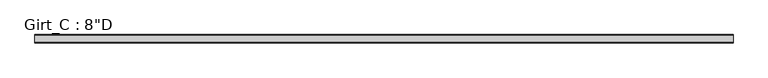
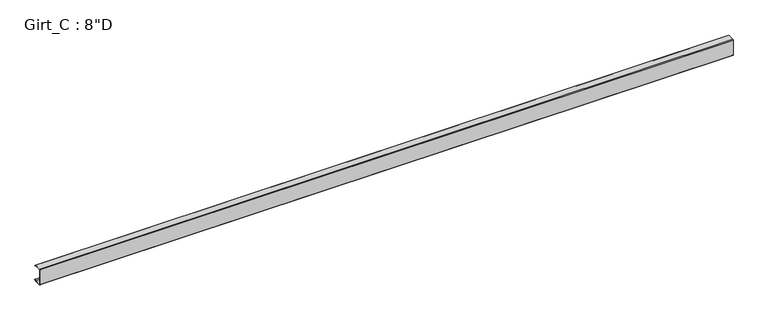
"""IFC4 building model written with IfcOpenShell, lengths in millimetres: beam geometry."""

from ifc_helpers import new_model, si_unit, point, frame, frame_2d, origin, place, context, project, spatial, polyline, circle_curve, trimmed, segment, composite_curve, outline, extrude, source, transform, mapped, element, save


def beam_3fe9278c(model_context):
    return source(origin(), model_context, "Body", "SweptSolid", [
        extrude(outline(composite_curve([segment(polyline([(87.5109375, 101.6), (99.7560415, 87.0068534), (97.6278742, 85.221109), (86.2154765, 98.821875), (3.3005807, 98.821875)]), True, "CONTINUOUS"), segment(trimmed(circle_curve(frame_2d((3.3741066, 96.8381931)), 1.9850441), [point((3.3005807, 98.821875))], [point((1.3890625, 96.8381931))], True, "CARTESIAN"), True, "CONTINUOUS"), segment(polyline([(1.3890625, 96.8381931), (1.3890625, -96.8389339)]), True, "CONTINUOUS"), segment(trimmed(circle_curve(frame_2d((3.3748024, -96.8389339)), 1.9857399), [point((1.3890625, -96.8389339))], [point((3.2694106, -98.821875))], True, "CARTESIAN"), True, "CONTINUOUS"), segment(polyline([(3.2694106, -98.821875), (86.2154765, -98.821875), (97.6510975, -85.1934327), (99.7792647, -86.979177), (87.5109375, -101.6), (3.3734375, -101.6)]), True, "CONTINUOUS"), segment(trimmed(circle_curve(frame_2d((3.3734375, -96.8375)), 4.7625), [point((3.3734375, -101.6))], [point((-1.3890625, -96.8375))], False, "CARTESIAN"), True, "CONTINUOUS"), segment(polyline([(-1.3890625, -96.8375), (-1.3890625, 96.8375)]), True, "CONTINUOUS"), segment(trimmed(circle_curve(frame_2d((3.3734375, 96.8375)), 4.7625), [point((-1.3890625, 96.8375))], [point((3.3734375, 101.6))], False, "CARTESIAN"), True, "CONTINUOUS"), segment(polyline([(3.3734375, 101.6), (87.5109375, 101.6)]), True, "CONTINUOUS")], self_intersect=False)), frame((-4206.5723786, 0.0, 0.0), z_axis=(1.0, 0.0, 0.0), x_axis=(0.0, 1.0, 0.0)), (0.0, 0.0, 1.0), 8444.8947573),
    ])


if __name__ == "__main__":
    model = new_model("IFC4")
    model_context = context("Model", 3, world=origin())
    ifc_project = project(units=[si_unit("LENGTHUNIT", "METRE", prefix="MILLI")], contexts=[model_context])
    site = spatial("IfcSite", under=ifc_project)
    building = spatial("IfcBuilding", under=site)
    placement = place(None, origin())
    beam_shape = beam_3fe9278c(model_context)
    element("IfcBeam", 1, ObjectType="Girt_C : 8\"D", at=placement, inside=building, context=model_context, shape_type="MappedRepresentation", body=[
        mapped(beam_shape, transform((0.0, 0.0, 0.0), x_axis=(1.0, 0.0, 0.0), y_axis=(0.0, 1.0, 0.0), z_axis=(0.0, 0.0, 1.0))),
    ])
    save(model, "model.ifc")

# Revit data of these elements
# Type "Girt_C : 8\"D"
#   half leg = 0' - 1 3/4"
#   Web_Thickness = 0' - 0 7/64"
#   Length [instance default] = 10' - 0"
#   Leg_1 = 0' - 3 1/2"
#   Height = 0' - 8"
#   Structural Material [instance default] = none
# Element 1 (IfcBeam, "Girt_C : 8\"D")
#   Structural Material = GALVANIZED 'CEE' SECTION (8.0x3.5C - SEE STRUCT. DWGS)
#   Materials on its faces: "GALVANIZED 'CEE' SECTION (8.0x3.5C - SEE STRUCT. DWGS)"
# Materials
#   "GALVANIZED 'CEE' SECTION (8.0x3.5C - SEE STRUCT. DWGS)": class "Metal", colour RGB 137 146 153, transparency 0, Description = "Steel, mill finish", Cost = 0
